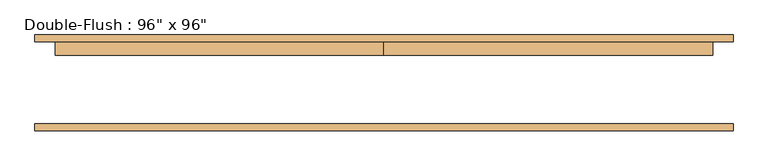
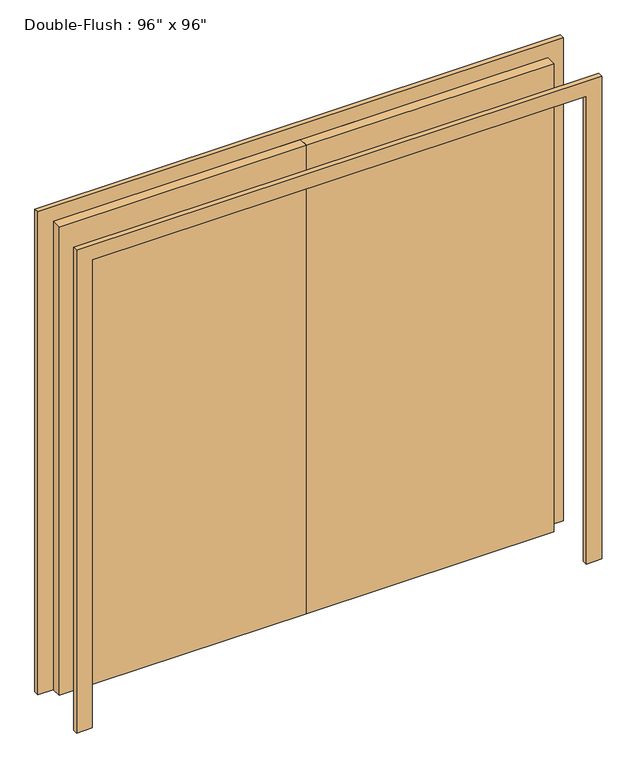
"""IFC4 building model written with IfcOpenShell, lengths in millimetres: door geometry."""

import ifcopenshell
import ifcopenshell.guid

model = None  # the IFC model being written
_history = None  # IfcOwnerHistory: only IFC2X3 demands one
_inside = {}  # id of a spatial element -> (the spatial element, [elements in it])
_under = {}  # id of a project, library or spatial element -> (it, [spatial elements below it])
_declared = {}  # id of a project -> (the project, [libraries it declares])
_typed = {}  # id of a type object -> (the type object, [elements of that type])
_made_of = {}  # id of a material, layer set ... -> (it, [elements and type objects made of it])


def new_model(schema):
    """Start an empty IFC model of exactly this schema.

    Asked for "IFC4X3", IfcOpenShell would pick the latest addendum, in which some entities
    have other attributes; the version numbers below select the first issue.
    IFC2X3 requires an IfcOwnerHistory on every rooted entity: one is made here for all.
    """
    global model, _history
    if schema == "IFC4X3":
        model = ifcopenshell.file(schema_version=(4, 3, 0, 0))
    else:
        model = ifcopenshell.file(schema=schema)
    _inside.clear()
    _under.clear()
    _declared.clear()
    _typed.clear()
    _made_of.clear()
    _history = None
    if model.schema == "IFC2X3":
        org = make("IfcOrganization", Name="unknown")
        user = make(
            "IfcPersonAndOrganization",
            ThePerson=make("IfcPerson", FamilyName="unknown"),
            TheOrganization=org,
        )
        app = make(
            "IfcApplication",
            ApplicationDeveloper=org,
            Version="unknown",
            ApplicationFullName="unknown",
            ApplicationIdentifier="unknown",
        )
        _history = make(
            "IfcOwnerHistory",
            OwningUser=user,
            OwningApplication=app,
            ChangeAction="ADDED",
            CreationDate=0,
        )
    return model


def make(cls, **values):
    """One entity of the class cls with the attributes given. An attribute that is None is left unset."""
    return model.create_entity(
        cls, **{name: value for name, value in values.items() if value is not None}
    )


def rooted(cls, **values):
    """An entity with a GlobalId (a new one), such as an element, a storey or a relation."""
    return make(cls, GlobalId=ifcopenshell.guid.new(), OwnerHistory=_history, **values)


def si_unit(unit_type, name, prefix=None):
    """IfcSIUnit, for example si_unit("LENGTHUNIT", "METRE", prefix="MILLI")."""
    return make("IfcSIUnit", UnitType=unit_type, Prefix=prefix, Name=name)


def assignment(units):
    """IfcUnitAssignment: the units of a project."""
    return None if units is None else make("IfcUnitAssignment", Units=units)


def point(xyz):
    """IfcCartesianPoint."""
    return None if xyz is None else make("IfcCartesianPoint", Coordinates=xyz)


def direction(xyz):
    """IfcDirection."""
    return None if xyz is None else make("IfcDirection", DirectionRatios=xyz)


def frame(location, z_axis=None, x_axis=None):
    """IfcAxis2Placement3D, a coordinate frame: its origin and axes. An axis left out is left unset."""
    return make(
        "IfcAxis2Placement3D",
        Location=point(location),
        Axis=direction(z_axis),
        RefDirection=direction(x_axis),
    )


def origin():
    """The frame at (0, 0, 0) with its axes left unset."""
    return frame((0.0, 0.0, 0.0))


def origin_with_axes():
    """The frame at (0, 0, 0) with the z axis (0, 0, 1) and the x axis (1, 0, 0) written out."""
    return frame((0.0, 0.0, 0.0), z_axis=(0.0, 0.0, 1.0), x_axis=(1.0, 0.0, 0.0))


def place(relative_to, where):
    """IfcLocalPlacement: puts the frame where relative to a parent placement (None: the world)."""
    return make(
        "IfcLocalPlacement", PlacementRelTo=relative_to, RelativePlacement=where
    )


def context(
    kind, dimensions, precision=None, world=None, true_north=None, identifier=None
):
    """IfcGeometricRepresentationContext, for example the 3D "Model" context."""
    return make(
        "IfcGeometricRepresentationContext",
        ContextIdentifier=identifier,
        ContextType=kind,
        CoordinateSpaceDimension=dimensions,
        Precision=precision,
        WorldCoordinateSystem=world,
        TrueNorth=true_north,
    )


def project(units=None, contexts=None):
    """IfcProject with its units and contexts."""
    return rooted(
        "IfcProject",
        Name="project",
        RepresentationContexts=contexts,
        UnitsInContext=assignment(units),
    )


def spatial(cls, under=None, at=None, **own):
    """A site, building, storey or space (cls), placed at a placement, below another one or the project."""
    s = rooted(cls, ObjectPlacement=at, **own)
    if under is not None:
        _under.setdefault(under.id(), (under, []))[1].append(s)
    return s


def polyline(points):
    """IfcPolyline through the points."""
    return make("IfcPolyline", Points=[point(p) for p in points])


def outline(outer, holes=None, kind="AREA"):
    """IfcArbitraryClosedProfileDef: a profile drawn as a closed curve; with holes, ...WithVoids."""
    if holes is None:
        return make("IfcArbitraryClosedProfileDef", ProfileType=kind, OuterCurve=outer)
    return make(
        "IfcArbitraryProfileDefWithVoids",
        ProfileType=kind,
        OuterCurve=outer,
        InnerCurves=holes,
    )


def extrude(swept, where, along, depth):
    """IfcExtrudedAreaSolid: the profile swept, set in the frame where, extruded along a direction by depth."""
    return make(
        "IfcExtrudedAreaSolid",
        SweptArea=swept,
        Position=where,
        ExtrudedDirection=direction(along),
        Depth=depth,
    )


def shape(context_of_items, identifier, shape_type, items):
    """IfcShapeRepresentation: the items that make up one representation, for example the "Body"."""
    return make(
        "IfcShapeRepresentation",
        ContextOfItems=context_of_items,
        RepresentationIdentifier=identifier,
        RepresentationType=shape_type,
        Items=items,
    )


def source(mapping_origin, context_of_items, identifier, shape_type, items):
    """IfcRepresentationMap: a shape defined once, which mapped items show again and again."""
    return make(
        "IfcRepresentationMap",
        MappingOrigin=mapping_origin,
        MappedRepresentation=shape(context_of_items, identifier, shape_type, items),
    )


def transform(
    local_origin,
    x_axis=None,
    y_axis=None,
    z_axis=None,
    scale=None,
    scale2=None,
    scale3=None,
    uniform=True,
):
    """IfcCartesianTransformationOperator3D, or its non-uniform kind. x_axis, y_axis, z_axis: its Axis1, 2, 3."""
    if uniform:
        return make(
            "IfcCartesianTransformationOperator3D",
            Axis1=direction(x_axis),
            Axis2=direction(y_axis),
            LocalOrigin=point(local_origin),
            Scale=scale,
            Axis3=direction(z_axis),
        )
    return make(
        "IfcCartesianTransformationOperator3DnonUniform",
        Axis1=direction(x_axis),
        Axis2=direction(y_axis),
        LocalOrigin=point(local_origin),
        Scale=scale,
        Axis3=direction(z_axis),
        Scale2=scale2,
        Scale3=scale3,
    )


def mapped(mapping_source, mapping_target):
    """IfcMappedItem: shows the shape of a source again, moved by a transform."""
    return make(
        "IfcMappedItem", MappingSource=mapping_source, MappingTarget=mapping_target
    )


def made_of(thing, what):
    """Note that an element or type object is made of a material, layer set ...; save() writes the relation."""
    if what is not None:
        _made_of.setdefault(what.id(), (what, []))[1].append(thing)
    return thing


def element(
    cls,
    number,
    at=None,
    inside=None,
    cuts=None,
    type_object=None,
    material=None,
    context=None,
    identifier="Body",
    shape_type=None,
    held_by="IfcProductDefinitionShape",
    body=None,
    shapes=None,
    **own,
):
    """One element of the class cls, such as IfcWall. Its Tag is "e" and its number.

    at: its placement. inside: the storey or other place that contains it. cuts: it is an
    opening in that element (IfcRelVoidsElement). A single representation is given by context,
    identifier, shape_type and body (its items); several are given by shapes. held_by: the class
    of the entity that holds the representations. save() writes the other relations.
    """
    e = rooted(cls, Tag="e%d" % number, ObjectPlacement=at, **own)
    if body is not None:
        shapes = [shape(context, identifier, shape_type, body)]
    if shapes is not None:
        e.Representation = make(held_by, Representations=shapes)
    if inside is not None:
        _inside.setdefault(inside.id(), (inside, []))[1].append(e)
    if cuts is not None:
        rooted(
            "IfcRelVoidsElement", RelatingBuildingElement=cuts, RelatedOpeningElement=e
        )
    if type_object is not None:
        _typed.setdefault(type_object.id(), (type_object, []))[1].append(e)
    return made_of(e, material)


def aggregate(whole, parts):
    """IfcRelAggregates: a whole, such as a stair, and the parts it consists of."""
    return rooted("IfcRelAggregates", RelatingObject=whole, RelatedObjects=parts)


def save(model, path):
    """Write the relations noted so far, then the file.

    IfcRelAggregates (storeys below a building ...), IfcRelContainedInSpatialStructure (elements
    in a storey), IfcRelDefinesByType, IfcRelAssociatesMaterial and IfcRelDeclares: one each for
    every whole, place, type object, material and project.
    """
    for whole, parts in _under.values():
        aggregate(whole, parts)
    for where, things in _inside.values():
        rooted(
            "IfcRelContainedInSpatialStructure",
            RelatedElements=things,
            RelatingStructure=where,
        )
    for kind, things in _typed.values():
        rooted("IfcRelDefinesByType", RelatedObjects=things, RelatingType=kind)
    for what, things in _made_of.values():
        rooted("IfcRelAssociatesMaterial", RelatedObjects=things, RelatingMaterial=what)
    for by, libraries in _declared.values():
        rooted("IfcRelDeclares", RelatingContext=by, RelatedDefinitions=libraries)
    model.write(path)


def door_656b4b26(model_context):
    return source(origin(), model_context, "Body", "SweptSolid", [
        extrude(outline(polyline([(0.0, 152.4), (1219.2, 152.4), (1219.2, 101.6), (0.0, 101.6), (0.0, 152.4)])), origin_with_axes(), (0.0, 0.0, 1.0), 2438.4),
        extrude(outline(polyline([(-1219.2, 152.4), (0.0, 152.4), (0.0, 101.6), (-1219.2, 101.6), (-1219.2, 152.4)])), origin_with_axes(), (0.0, 0.0, 1.0), 2438.4),
        extrude(outline(polyline([(2438.4, -1219.2), (2438.4, 1219.2), (0.0, 1219.2), (0.0, 1295.4), (2514.6, 1295.4), (2514.6, -1295.4), (0.0, -1295.4), (0.0, -1219.2), (2438.4, -1219.2)])), frame((0.0, -177.8, 0.0), z_axis=(0.0, 1.0, 0.0), x_axis=(0.0, 0.0, 1.0)), (0.0, 0.0, 1.0), 25.4),
        extrude(outline(polyline([(2438.4, -1219.2), (2438.4, 1219.2), (0.0, 1219.2), (0.0, 1295.4), (2514.6, 1295.4), (2514.6, -1295.4), (0.0, -1295.4), (0.0, -1219.2), (2438.4, -1219.2)])), frame((0.0, 152.4, 0.0), z_axis=(0.0, 1.0, 0.0), x_axis=(0.0, 0.0, 1.0)), (0.0, 0.0, 1.0), 25.4),
    ])


if __name__ == "__main__":
    model = new_model("IFC4")
    model_context = context("Model", 3, world=origin())
    ifc_project = project(units=[si_unit("LENGTHUNIT", "METRE", prefix="MILLI")], contexts=[model_context])
    site = spatial("IfcSite", under=ifc_project)
    building = spatial("IfcBuilding", under=site)
    placement = place(None, origin())
    door_shape = door_656b4b26(model_context)
    element("IfcDoor", 1, ObjectType="Double-Flush : 96\" x 96\"", at=placement, inside=building, context=model_context, shape_type="MappedRepresentation", body=[
        mapped(door_shape, transform((0.0, 0.0, 0.0), x_axis=(1.0, 0.0, 0.0), y_axis=(0.0, 1.0, 0.0), z_axis=(0.0, 0.0, 1.0))),
    ])
    save(model, "model.ifc")

# Revit data of these elements
# Type "Double-Flush : 96\" x 96\""
#   Type Mark = "39"
#   Assembly Code = "C1020"
#   Thickness = 50.8 mm
#   Height = 2438.4 mm
#   Trim Projection Ext = 25.4 mm
#   Trim Projection Int = 25.4 mm
#   Trim Width = 76.2 mm
#   Width = 2438.4 mm
#   Door Material = Door - Panel
#   Frame Material = Door - Frame
#   Function = (empty or 0)
#   Wall Closure = (empty or 0)
# Element 1 (IfcDoor, "Double-Flush : 96\" x 96\"")
#   Materials on its faces: "Door - Frame", "Door - Panel"
# Materials
#   "Door - Panel": class "Wood", colour RGB 210 159 95, transparency 0
#   "Door - Frame": class "Miscellaneous", colour RGB 118 70 51, transparency 0
